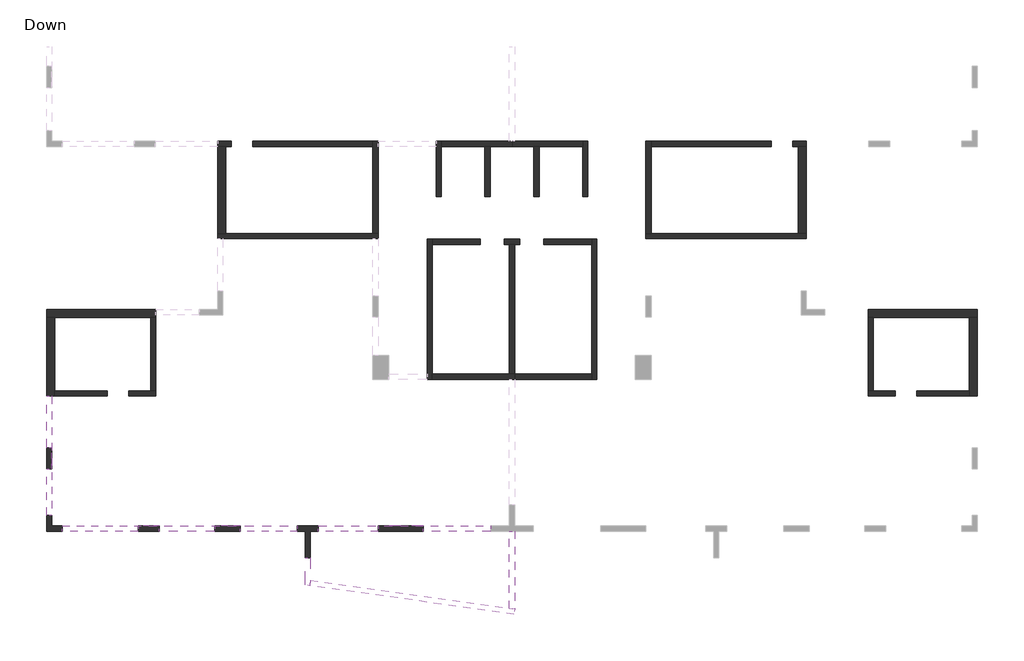
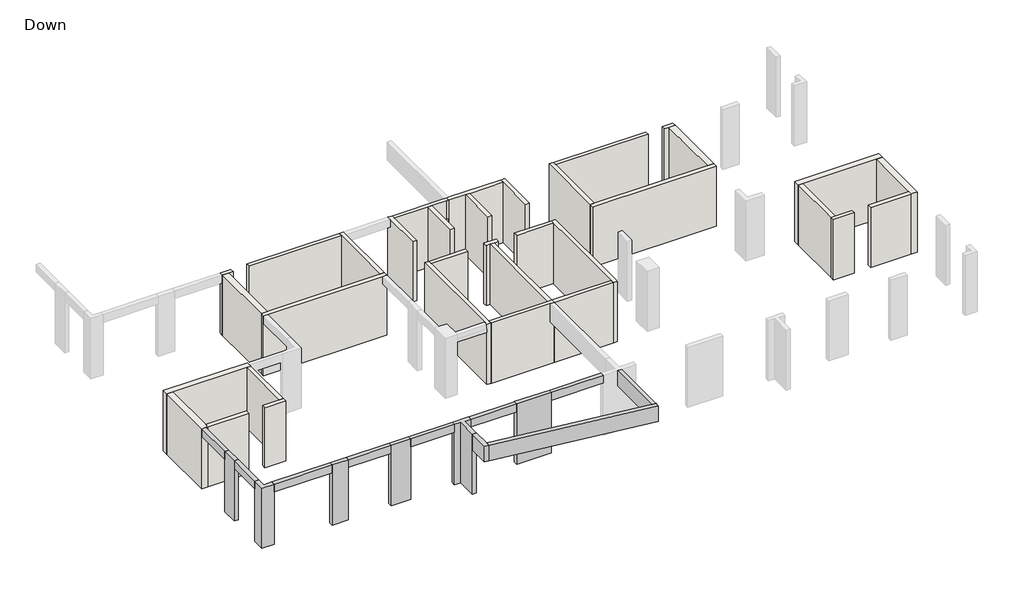
# One storey, part 1 of 2: 34 walls, 10 beams, 6 columns.
# Revit data of these elements (continued)
# Element 25 (IfcWall, "20") (continued)
#   SOFiSTiK_EdgeZones = "W15"
#   SOFiSTiK_AMG_Comments = ""
#   Top Offset = 0 cm
#   Base Offset = 0 cm
#   wall height = 312 cm
#   SOFiSTiK_AMG_Scheduled = yes
#   SOFiSTiK_AMG_Adjusted = yes
#   Phase Created = New Construction
#   Base Constraint = Down
#   Top Constraint = Typical Floor
#   Materials on its faces: "Concrete"
# Element 26 (IfcWall, "20")
#   Comments = ""
#   Mark = "W22"
#   SOFiSTiK_EdgeZones = "W16"
#   SOFiSTiK_AMG_Comments = ""
#   Top Offset = 0 cm
#   Base Offset = 0 cm
#   wall height = 312 cm
#   SOFiSTiK_AMG_Scheduled = yes
#   SOFiSTiK_AMG_Adjusted = yes
#   Phase Created = New Construction
#   Base Constraint = Down
#   Top Constraint = Typical Floor
#   Materials on its faces: "Concrete"
# Element 27 (IfcWall, "20")
#   Comments = ""
#   Mark = "W23"
#   SOFiSTiK_EdgeZones = "W17"
#   SOFiSTiK_AMG_Comments = ""
#   Top Offset = 0 cm
#   Base Offset = 0 cm
#   wall height = 312 cm
#   SOFiSTiK_AMG_Scheduled = yes
#   SOFiSTiK_AMG_Adjusted = yes
#   Phase Created = New Construction
#   Base Constraint = Down
#   Top Constraint = Typical Floor
#   Materials on its faces: "Concrete"
# Element 28 (IfcWall, "20")
#   Comments = ""
#   Mark = "W24"
#   SOFiSTiK_EdgeZones = "W18"
#   SOFiSTiK_AMG_Comments = ""
#   Top Offset = 0 cm
#   Base Offset = 0 cm
#   wall height = 312 cm
#   SOFiSTiK_AMG_Scheduled = yes
#   SOFiSTiK_AMG_Adjusted = yes
#   Phase Created = New Construction
#   Base Constraint = Down
#   Top Constraint = Typical Floor
#   Materials on its faces: "Concrete"
# Element 29 (IfcWall, "20")
#   Comments = ""
#   Mark = "W25"
#   SOFiSTiK_EdgeZones = "W19"
#   SOFiSTiK_AMG_Comments = ""
#   Top Offset = 0 cm
#   Base Offset = 0 cm
#   wall height = 312 cm
#   SOFiSTiK_AMG_Scheduled = yes
#   SOFiSTiK_AMG_Adjusted = yes
#   Phase Created = New Construction
#   Base Constraint = Down
#   Top Constraint = Typical Floor
#   Materials on its faces: "Concrete"
# Element 30 (IfcWall, "20")
#   Comments = ""
#   Mark = "W26"
#   SOFiSTiK_EdgeZones = "W20"
#   SOFiSTiK_AMG_Comments = ""
#   Top Offset = 0 cm
#   Base Offset = 0 cm
#   wall height = 312 cm
#   SOFiSTiK_AMG_Scheduled = yes
#   SOFiSTiK_AMG_Adjusted = yes
#   Phase Created = New Construction
#   Base Constraint = Down
#   Top Constraint = Typical Floor
#   Materials on its faces: "Concrete"
# Element 31 (IfcWall, "20")
#   Comments = ""
#   Mark = "W27"
#   SOFiSTiK_EdgeZones = "W21"
#   SOFiSTiK_AMG_Comments = ""
#   Top Offset = 0 cm
#   Base Offset = 0 cm
#   wall height = 312 cm
#   SOFiSTiK_AMG_Scheduled = yes
#   SOFiSTiK_AMG_Adjusted = yes
#   Phase Created = New Construction
#   Base Constraint = Down
#   Top Constraint = Typical Floor
#   Materials on its faces: "Concrete"
# Element 32 (IfcWall, "20")
#   Comments = ""
#   Mark = "W28"
#   SOFiSTiK_EdgeZones = "W22"
#   SOFiSTiK_AMG_Comments = ""
#   Top Offset = 0 cm
#   Base Offset = 0 cm
#   wall height = 312 cm
#   SOFiSTiK_AMG_Scheduled = yes
#   SOFiSTiK_AMG_Adjusted = yes
#   Phase Created = New Construction
#   Base Constraint = Down
#   Top Constraint = Typical Floor
#   Materials on its faces: "Concrete"
# Element 33 (IfcWall, "20")
#   Comments = ""
#   Mark = "W29"
#   SOFiSTiK_EdgeZones = "W23"
#   SOFiSTiK_AMG_Comments = ""
#   Top Offset = 0 cm
#   Base Offset = 0 cm
#   wall height = 312 cm
#   SOFiSTiK_AMG_Scheduled = yes
#   SOFiSTiK_AMG_Adjusted = yes
#   Phase Created = New Construction
#   Base Constraint = Down
#   Top Constraint = Typical Floor
#   Materials on its faces: "Concrete"
# Element 34 (IfcWall, "20")
#   Comments = ""
#   Mark = "W30"
#   SOFiSTiK_EdgeZones = "W24"
#   SOFiSTiK_AMG_Comments = ""
#   Top Offset = 0 cm
#   Base Offset = 0 cm
#   wall height = 312 cm
#   SOFiSTiK_AMG_Scheduled = yes
#   SOFiSTiK_AMG_Adjusted = yes
#   Phase Created = New Construction
#   Base Constraint = Down
#   Top Constraint = Typical Floor
#   Materials on its faces: "Concrete"
# Element 35 (IfcWall, "20")
#   Comments = ""
#   Mark = "W31"
#   SOFiSTiK_EdgeZones = "W25"
#   SOFiSTiK_AMG_Comments = ""
#   Top Offset = 0 cm
#   Base Offset = 0 cm
#   wall height = 312 cm
#   SOFiSTiK_AMG_Scheduled = yes
#   SOFiSTiK_AMG_Adjusted = yes
#   Phase Created = New Construction
#   Base Constraint = Down
#   Top Constraint = Typical Floor
#   Materials on its faces: "Concrete"
# Element 36 (IfcWall, "20")
#   Comments = ""
#   Mark = "W32"
#   SOFiSTiK_EdgeZones = "W26"
#   SOFiSTiK_AMG_Comments = ""
#   Top Offset = 0 cm
#   Base Offset = 0 cm
#   wall height = 312 cm
#   SOFiSTiK_AMG_Scheduled = yes
#   SOFiSTiK_AMG_Adjusted = yes
#   Phase Created = New Construction
#   Base Constraint = Down
#   Top Constraint = Typical Floor
#   Materials on its faces: "Concrete"
# Element 37 (IfcWall, "20")
#   Comments = ""
#   Mark = "W33"
#   SOFiSTiK_EdgeZones = "W27"
#   SOFiSTiK_AMG_Comments = ""
#   Top Offset = 0 cm
#   Base Offset = 0 cm
#   wall height = 312 cm
#   SOFiSTiK_AMG_Scheduled = yes
#   SOFiSTiK_AMG_Adjusted = yes
#   Phase Created = New Construction
#   Base Constraint = Down
#   Top Constraint = Typical Floor
#   Materials on its faces: "Concrete"
# Element 38 (IfcWall, "20")
#   Comments = ""
#   Mark = "W34"
#   SOFiSTiK_EdgeZones = "W28"
#   SOFiSTiK_AMG_Comments = ""
#   Top Offset = 0 cm
#   Base Offset = 0 cm
#   wall height = 312 cm
#   SOFiSTiK_AMG_Scheduled = yes
#   SOFiSTiK_AMG_Adjusted = yes
#   Phase Created = New Construction
#   Base Constraint = Down
#   Top Constraint = Typical Floor
#   Materials on its faces: "Concrete"
# Element 39 (IfcWall, "20")
#   Comments = ""
#   Mark = "W35"
#   SOFiSTiK_EdgeZones = "W29"
#   SOFiSTiK_AMG_Comments = ""
#   Top Offset = 0 cm
#   Base Offset = 0 cm
#   wall height = 312 cm
#   SOFiSTiK_AMG_Scheduled = yes
#   SOFiSTiK_AMG_Adjusted = yes
#   Phase Created = New Construction
#   Base Constraint = Down
#   Top Constraint = Typical Floor
#   Materials on its faces: "Concrete"
# Element 40 (IfcWall, "20")
#   Comments = ""
#   Mark = "W36"
#   SOFiSTiK_EdgeZones = "W30"
#   SOFiSTiK_AMG_Comments = ""
#   Top Offset = 0 cm
#   Base Offset = 0 cm
#   wall height = 312 cm
#   SOFiSTiK_AMG_Scheduled = yes
#   SOFiSTiK_AMG_Adjusted = yes
#   Phase Created = New Construction
#   Base Constraint = Down
#   Top Constraint = Typical Floor
#   Materials on its faces: "Concrete"
# Element 41 (IfcWall, "20")
#   Comments = ""
#   Mark = "W37"
#   SOFiSTiK_EdgeZones = "W31"
#   SOFiSTiK_AMG_Comments = ""
#   Top Offset = 0 cm
#   Base Offset = 0 cm
#   wall height = 312 cm
#   SOFiSTiK_AMG_Scheduled = yes
#   SOFiSTiK_AMG_Adjusted = yes
#   Phase Created = New Construction
#   Base Constraint = Down
#   Top Constraint = Typical Floor
#   Materials on its faces: "Concrete"
# Element 42 (IfcWall, "20")
#   Comments = ""
#   Mark = "W39"
#   SOFiSTiK_EdgeZones = "W32"
#   SOFiSTiK_AMG_Comments = ""
#   Top Offset = 0 cm
#   Base Offset = 0 cm
#   wall height = 312 cm
#   SOFiSTiK_AMG_Scheduled = yes
#   SOFiSTiK_AMG_Adjusted = yes
#   Phase Created = New Construction
#   Base Constraint = Down
#   Top Constraint = Typical Floor
#   Materials on its faces: "Concrete"
# Element 43 (IfcWall, "20")
#   Comments = ""
#   Mark = "W40"
#   SOFiSTiK_EdgeZones = "W33"
#   SOFiSTiK_AMG_Comments = ""
#   Top Offset = 0 cm
#   Base Offset = 0 cm
#   wall height = 312 cm
#   SOFiSTiK_AMG_Scheduled = yes
#   SOFiSTiK_AMG_Adjusted = yes
#   Phase Created = New Construction
#   Base Constraint = Down
#   Top Constraint = Typical Floor
#   Materials on its faces: "Concrete"
# Element 44 (IfcWall, "20")
#   Comments = ""
#   Mark = "W41"
#   SOFiSTiK_EdgeZones = "W34"
#   SOFiSTiK_AMG_Comments = ""
#   Top Offset = 0 cm
#   Base Offset = 0 cm
#   wall height = 312 cm
#   SOFiSTiK_AMG_Scheduled = yes
#   SOFiSTiK_AMG_Adjusted = yes
#   Phase Created = New Construction
#   Base Constraint = Down
#   Top Constraint = Typical Floor
#   Materials on its faces: "Concrete"
# Element 45 (IfcWall, "30")
#   Comments = ""
#   Mark = "W1"
#   SOFiSTiK_EdgeZones = "W1"
#   SOFiSTiK_AMG_Comments = ""
#   Top Offset = 0 cm
#   Base Offset = 0 cm
#   wall height = 312 cm
#   SOFiSTiK_AMG_Scheduled = yes
#   SOFiSTiK_AMG_Adjusted = yes
#   Phase Created = New Construction
#   Base Constraint = Down
#   Top Constraint = Typical Floor
#   Materials on its faces: "Concrete"
# Element 46 (IfcWall, "30")
#   Comments = ""
#   Mark = "W2"
#   SOFiSTiK_EdgeZones = "W2"
#   SOFiSTiK_AMG_Comments = ""
#   Top Offset = 0 cm
#   Base Offset = 0 cm
#   wall height = 312 cm
#   SOFiSTiK_AMG_Scheduled = yes
#   SOFiSTiK_AMG_Adjusted = yes
#   Phase Created = New Construction
#   Base Constraint = Down
#   Top Constraint = Typical Floor
#   Materials on its faces: "Concrete"
# Element 47 (IfcWall, "30")
#   Comments = ""
#   Mark = "W3"
#   SOFiSTiK_EdgeZones = "W3"
#   SOFiSTiK_AMG_Comments = ""
#   Top Offset = 0 cm
#   Base Offset = 0 cm
#   wall height = 312 cm
#   SOFiSTiK_AMG_Scheduled = yes
#   SOFiSTiK_AMG_Adjusted = yes
#   Phase Created = New Construction
#   Base Constraint = Down
#   Top Constraint = Typical Floor
#   Materials on its faces: "Concrete"
# Element 48 (IfcWall, "30")
#   Comments = ""
#   Mark = "W4"
#   SOFiSTiK_EdgeZones = "W4"
#   SOFiSTiK_AMG_Comments = ""
#   Top Offset = 0 cm
#   Base Offset = 0 cm
#   wall height = 312 cm
#   SOFiSTiK_AMG_Scheduled = yes
#   SOFiSTiK_AMG_Adjusted = yes
#   Phase Created = New Construction
#   Base Constraint = Down
#   Top Constraint = Typical Floor
#   Materials on its faces: "Concrete"
# Element 49 (IfcWall, "30")
#   Comments = ""
#   Mark = "W5"
#   SOFiSTiK_EdgeZones = "W5"
#   SOFiSTiK_AMG_Comments = ""
#   Top Offset = 0 cm
#   Base Offset = 0 cm
#   wall height = 312 cm
#   SOFiSTiK_AMG_Scheduled = yes
#   SOFiSTiK_AMG_Adjusted = yes
#   Phase Created = New Construction
#   Base Constraint = Down
#   Top Constraint = Typical Floor
#   Materials on its faces: "Concrete"
# Element 50 (IfcWall, "30")
#   Comments = ""
#   Mark = "W6"
#   SOFiSTiK_EdgeZones = "W6"
#   SOFiSTiK_AMG_Comments = ""
#   Top Offset = 0 cm
#   Base Offset = 0 cm
#   wall height = 312 cm
#   SOFiSTiK_AMG_Scheduled = yes
#   SOFiSTiK_AMG_Adjusted = yes
#   Phase Created = New Construction
#   Base Constraint = Down
#   Top Constraint = Typical Floor
#   Materials on its faces: "Concrete"
# Materials
#   "Concrete": class "Concrete", colour RGB 192 192 192, transparency 0, Keynote = "01000", Description = "Cast-in-place concrete", Cost = 0
#   "Concrete, Cast-in-Place gray": class "Concrete", colour RGB 192 192 192, transparency 0, Description = "Cast-in-place concrete", Cost = 0
